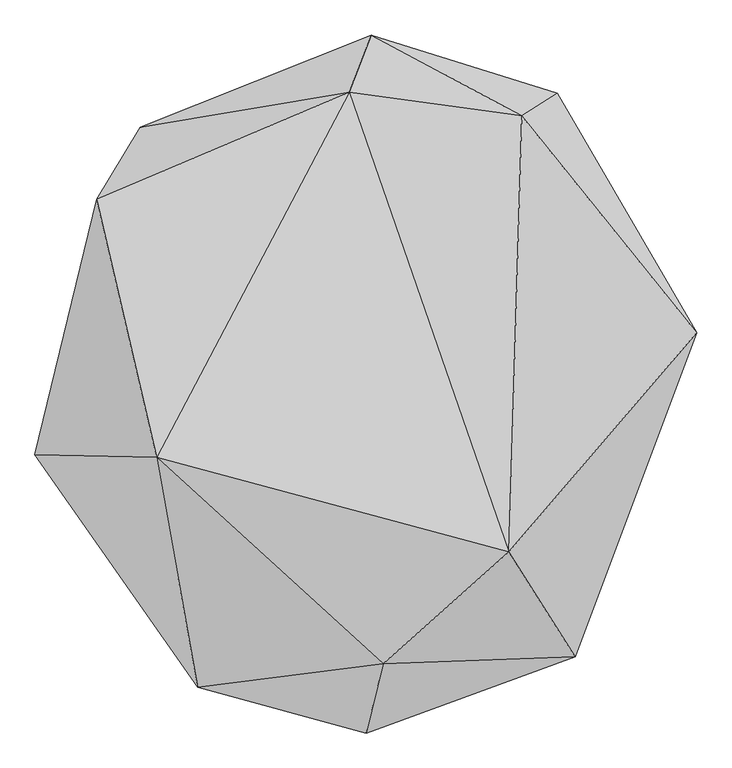
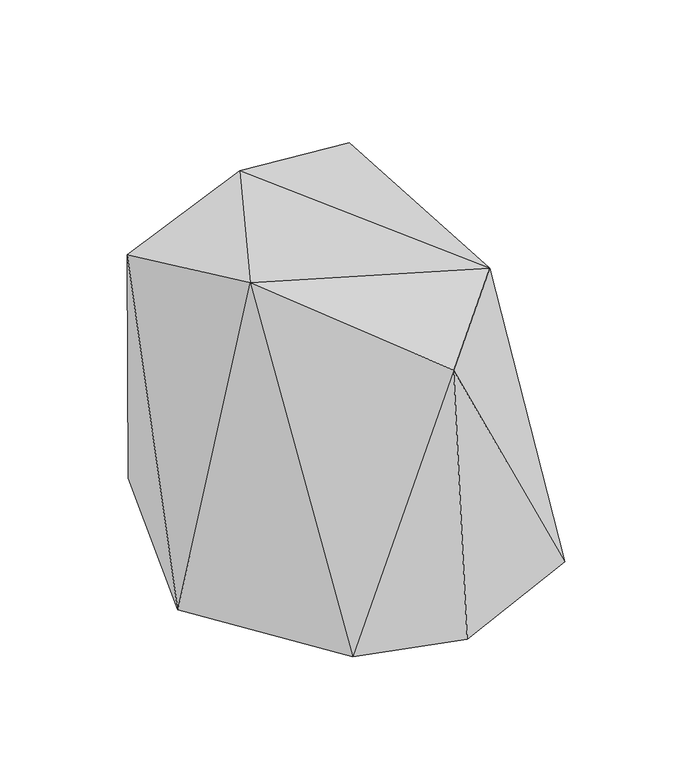
"""IFC4 building model written with IfcOpenShell, lengths in millimetres: geographic element geometry, Enscape AssetDefinition - Bush 124 Pampas Grass : Enscape AssetDefinition - Bush 124 Pampas Grass."""

from ifc_helpers import new_model, si_unit, origin, place, context, project, spatial, faceted_brep, source, transform, mapped, element, save


def geographic_element_9c8827ca(model_context):
    return source(origin(), model_context, "Body", "Brep", [
        faceted_brep([(-264.2639875, -536.5539789, 88.6489972), (-339.3009901, -117.5350025, 1082.6699734), (-560.995996, -112.7799973, 88.6489972), (11.8039995, 547.9059815, 923.6680269), (-448.6410022, 352.7109921, 928.7919998), (73.4319985, -493.712008, 881.5860152), (302.7119935, -289.655, 1010.3069544), (-369.4530129, 484.5449924, 88.6489972), (-107.4849963, -0.627, -7.4829999), (42.5710008, -619.6249723, 88.6449963), (423.4899879, -480.5459976, 124.5009974), (644.8199749, 109.6689999, 125.455007), (326.1559904, 504.7410131, 931.0209751), (52.0480014, 652.4310112, 88.6489972), (391.2200034, 546.1400151, 88.6489972)], [[[0, 1, 2]], [[3, 4, 1]], [[4, 2, 1]], [[0, 5, 1]], [[6, 3, 1]], [[5, 6, 1]], [[2, 7, 8]], [[2, 8, 0]], [[7, 2, 4]], [[0, 9, 5]], [[0, 8, 9]], [[10, 5, 9]], [[10, 6, 5]], [[11, 12, 6]], [[12, 3, 6]], [[10, 11, 6]], [[9, 8, 10]], [[10, 8, 11]], [[13, 14, 8]], [[8, 7, 13]], [[8, 14, 11]], [[13, 7, 3]], [[3, 7, 4]], [[14, 13, 12]], [[12, 13, 3]], [[11, 14, 12]]]),
    ])


if __name__ == "__main__":
    model = new_model("IFC4")
    model_context = context("Model", 3, world=origin())
    ifc_project = project(units=[si_unit("LENGTHUNIT", "METRE", prefix="MILLI")], contexts=[model_context])
    site = spatial("IfcSite", under=ifc_project)
    building = spatial("IfcBuilding", under=site)
    placement = place(None, origin())
    geographic_element_shape = geographic_element_9c8827ca(model_context)
    element("IfcGeographicElement", 1, ObjectType="Enscape AssetDefinition - Bush 124 Pampas Grass : Enscape AssetDefinition - Bush 124 Pampas Grass", at=placement, inside=building, context=model_context, shape_type="MappedRepresentation", body=[
        mapped(geographic_element_shape, transform((0.0, 0.0, 0.0), x_axis=(1.0, 0.0, 0.0), y_axis=(0.0, 1.0, 0.0), z_axis=(0.0, 0.0, 1.0))),
    ])
    save(model, "model.ifc")

# Revit data of these elements
# Type "Enscape AssetDefinition - Bush 124 Pampas Grass : Enscape AssetDefinition - Bush 124 Pampas Grass"
#   EnscapeAssetSource = "REMOTE"
#   EnscapeAssetId = "c051ca4c-e4a4-4b28-9467-8725a50cb4a2"
#   Height = 1.08267 m
#   EnscapeNativeAssetHeight = 1.08267 m
#   Default Elevation = 0
